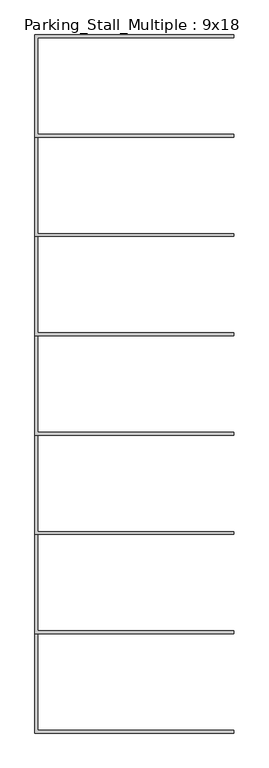
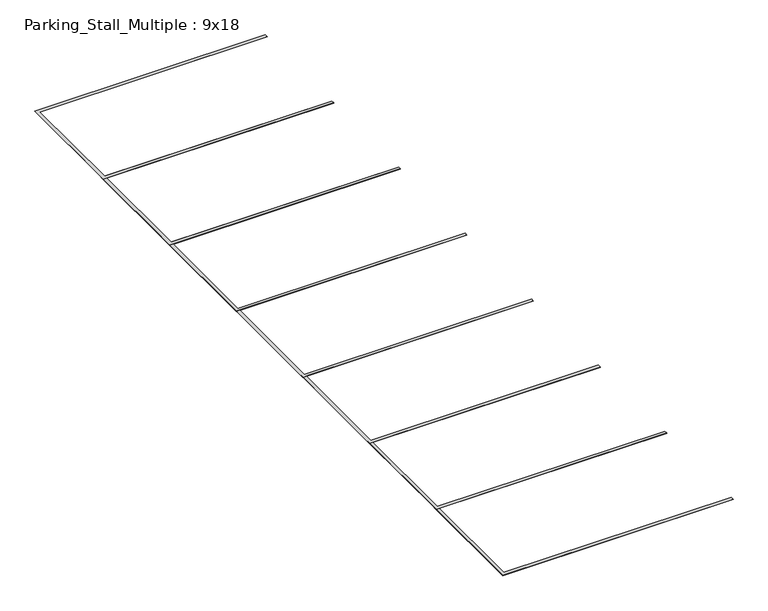
"""IFC4 building model written with IfcOpenShell, lengths in millimetres: proxy geometry, Parking_Stall_Multiple : 9x18."""

from ifc_helpers import new_model, si_unit, origin, origin_with_axes, place, context, project, spatial, polyline, outline, extrude, source, transform, mapped, element, save


def parking_stall_multiple_9x18_ae039515(model_context):
    return source(origin(), model_context, "Body", "SweptSolid", [
        extrude(outline(polyline([(5486.4, 16459.2), (0.0, 16459.2), (0.0, 19278.6), (5486.4, 19278.6), (5486.4, 19202.4), (76.2, 19202.4), (76.2, 16535.4), (5486.4, 16535.4), (5486.4, 16459.2)])), origin_with_axes(), (0.0, 0.0, 1.0), 6.35),
        extrude(outline(polyline([(5486.4, 13716.0), (0.0, 13716.0), (0.0, 16535.4), (5486.4, 16535.4), (5486.4, 16459.2), (76.2, 16459.2), (76.2, 13792.2), (5486.4, 13792.2), (5486.4, 13716.0)])), origin_with_axes(), (0.0, 0.0, 1.0), 6.35),
        extrude(outline(polyline([(5486.4, 10972.8), (0.0, 10972.8), (0.0, 13792.2), (5486.4, 13792.2), (5486.4, 13716.0), (76.2, 13716.0), (76.2, 11049.0), (5486.4, 11049.0), (5486.4, 10972.8)])), origin_with_axes(), (0.0, 0.0, 1.0), 6.35),
        extrude(outline(polyline([(5486.4, 8229.6), (0.0, 8229.6), (0.0, 11049.0), (5486.4, 11049.0), (5486.4, 10972.8), (76.2, 10972.8), (76.2, 8305.8), (5486.4, 8305.8), (5486.4, 8229.6)])), origin_with_axes(), (0.0, 0.0, 1.0), 6.35),
        extrude(outline(polyline([(5486.4, 5486.4), (0.0, 5486.4), (0.0, 8305.8), (5486.4, 8305.8), (5486.4, 8229.6), (76.2, 8229.6), (76.2, 5562.6), (5486.4, 5562.6), (5486.4, 5486.4)])), origin_with_axes(), (0.0, 0.0, 1.0), 6.35),
        extrude(outline(polyline([(5486.4, 2743.2), (0.0, 2743.2), (0.0, 5562.6), (5486.4, 5562.6), (5486.4, 5486.4), (76.2, 5486.4), (76.2, 2819.4), (5486.4, 2819.4), (5486.4, 2743.2)])), origin_with_axes(), (0.0, 0.0, 1.0), 6.35),
        extrude(outline(polyline([(5486.4, 0.0), (0.0, 0.0), (0.0, 2819.4), (5486.4, 2819.4), (5486.4, 2743.2), (76.2, 2743.2), (76.2, 76.2), (5486.4, 76.2), (5486.4, 0.0)])), origin_with_axes(), (0.0, 0.0, 1.0), 6.35),
    ])


if __name__ == "__main__":
    model = new_model("IFC4")
    model_context = context("Model", 3, world=origin())
    ifc_project = project(units=[si_unit("LENGTHUNIT", "METRE", prefix="MILLI")], contexts=[model_context])
    site = spatial("IfcSite", under=ifc_project)
    building = spatial("IfcBuilding", under=site)
    placement = place(None, origin())
    parking_stall_multiple_9x18_shape = parking_stall_multiple_9x18_ae039515(model_context)
    element("IfcBuildingElementProxy", 1, Name="Parking_Stall_Multiple : 9x18", ObjectType="Parking_Stall_Multiple : 9x18", at=placement, inside=building, context=model_context, shape_type="MappedRepresentation", body=[
        mapped(parking_stall_multiple_9x18_shape, transform((0.0, 0.0, 0.0), x_axis=(1.0, 0.0, 0.0), y_axis=(0.0, 1.0, 0.0), z_axis=(0.0, 0.0, 1.0))),
    ])
    save(model, "model.ifc")

# Revit data of these elements
# Type "Parking_Stall_Multiple : 9x18"
#   Parking_Width_M = 9' - 0"
#   Parking_Run_Length [instance default] = 65' - 0"
#   Parking_Length_M = 18' - 0"
#   Single_Parking_Visibility [instance default] = no
#   ParkingUnitsArray [instance default] = 7
#   ParkingUnits [instance default] = 7
#   Multiple_Parking_Visibility [instance default] = yes
